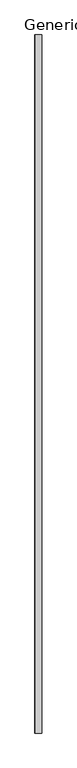
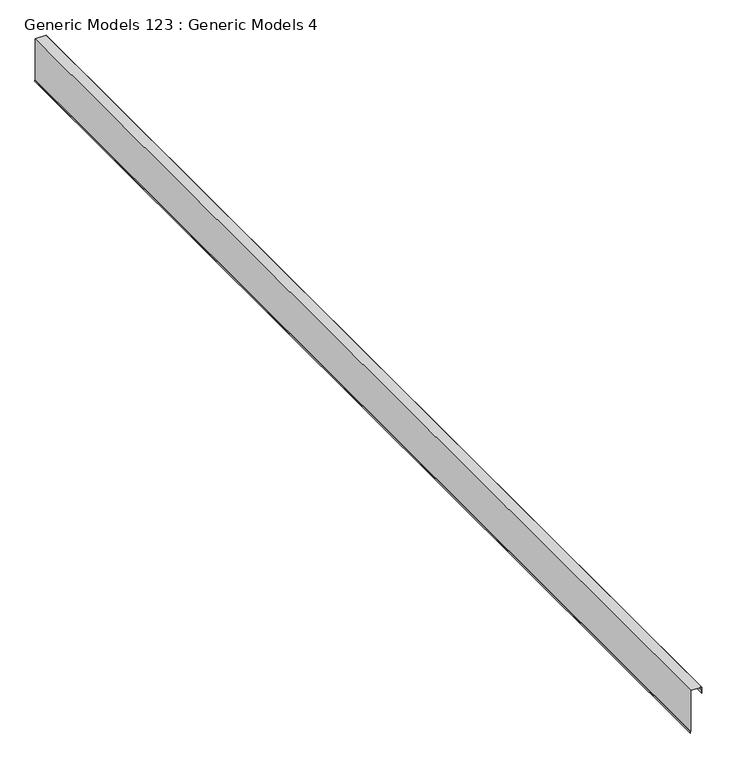
"""IFC4 building model written with IfcOpenShell, lengths in millimetres: proxy geometry, Generic Models 123 : Generic Models 4."""

import ifcopenshell
import ifcopenshell.guid

model = None  # the IFC model being written
_history = None  # IfcOwnerHistory: only IFC2X3 demands one
_inside = {}  # id of a spatial element -> (the spatial element, [elements in it])
_under = {}  # id of a project, library or spatial element -> (it, [spatial elements below it])
_declared = {}  # id of a project -> (the project, [libraries it declares])
_typed = {}  # id of a type object -> (the type object, [elements of that type])
_made_of = {}  # id of a material, layer set ... -> (it, [elements and type objects made of it])


def new_model(schema):
    """Start an empty IFC model of exactly this schema.

    Asked for "IFC4X3", IfcOpenShell would pick the latest addendum, in which some entities
    have other attributes; the version numbers below select the first issue.
    IFC2X3 requires an IfcOwnerHistory on every rooted entity: one is made here for all.
    """
    global model, _history
    if schema == "IFC4X3":
        model = ifcopenshell.file(schema_version=(4, 3, 0, 0))
    else:
        model = ifcopenshell.file(schema=schema)
    _inside.clear()
    _under.clear()
    _declared.clear()
    _typed.clear()
    _made_of.clear()
    _history = None
    if model.schema == "IFC2X3":
        org = make("IfcOrganization", Name="unknown")
        user = make(
            "IfcPersonAndOrganization",
            ThePerson=make("IfcPerson", FamilyName="unknown"),
            TheOrganization=org,
        )
        app = make(
            "IfcApplication",
            ApplicationDeveloper=org,
            Version="unknown",
            ApplicationFullName="unknown",
            ApplicationIdentifier="unknown",
        )
        _history = make(
            "IfcOwnerHistory",
            OwningUser=user,
            OwningApplication=app,
            ChangeAction="ADDED",
            CreationDate=0,
        )
    return model


def make(cls, **values):
    """One entity of the class cls with the attributes given. An attribute that is None is left unset."""
    return model.create_entity(
        cls, **{name: value for name, value in values.items() if value is not None}
    )


def rooted(cls, **values):
    """An entity with a GlobalId (a new one), such as an element, a storey or a relation."""
    return make(cls, GlobalId=ifcopenshell.guid.new(), OwnerHistory=_history, **values)


def si_unit(unit_type, name, prefix=None):
    """IfcSIUnit, for example si_unit("LENGTHUNIT", "METRE", prefix="MILLI")."""
    return make("IfcSIUnit", UnitType=unit_type, Prefix=prefix, Name=name)


def assignment(units):
    """IfcUnitAssignment: the units of a project."""
    return None if units is None else make("IfcUnitAssignment", Units=units)


def point(xyz):
    """IfcCartesianPoint."""
    return None if xyz is None else make("IfcCartesianPoint", Coordinates=xyz)


def direction(xyz):
    """IfcDirection."""
    return None if xyz is None else make("IfcDirection", DirectionRatios=xyz)


def frame(location, z_axis=None, x_axis=None):
    """IfcAxis2Placement3D, a coordinate frame: its origin and axes. An axis left out is left unset."""
    return make(
        "IfcAxis2Placement3D",
        Location=point(location),
        Axis=direction(z_axis),
        RefDirection=direction(x_axis),
    )


def origin():
    """The frame at (0, 0, 0) with its axes left unset."""
    return frame((0.0, 0.0, 0.0))


def place(relative_to, where):
    """IfcLocalPlacement: puts the frame where relative to a parent placement (None: the world)."""
    return make(
        "IfcLocalPlacement", PlacementRelTo=relative_to, RelativePlacement=where
    )


def context(
    kind, dimensions, precision=None, world=None, true_north=None, identifier=None
):
    """IfcGeometricRepresentationContext, for example the 3D "Model" context."""
    return make(
        "IfcGeometricRepresentationContext",
        ContextIdentifier=identifier,
        ContextType=kind,
        CoordinateSpaceDimension=dimensions,
        Precision=precision,
        WorldCoordinateSystem=world,
        TrueNorth=true_north,
    )


def project(units=None, contexts=None):
    """IfcProject with its units and contexts."""
    return rooted(
        "IfcProject",
        Name="project",
        RepresentationContexts=contexts,
        UnitsInContext=assignment(units),
    )


def spatial(cls, under=None, at=None, **own):
    """A site, building, storey or space (cls), placed at a placement, below another one or the project."""
    s = rooted(cls, ObjectPlacement=at, **own)
    if under is not None:
        _under.setdefault(under.id(), (under, []))[1].append(s)
    return s


def polyline(points):
    """IfcPolyline through the points."""
    return make("IfcPolyline", Points=[point(p) for p in points])


def outline(outer, holes=None, kind="AREA"):
    """IfcArbitraryClosedProfileDef: a profile drawn as a closed curve; with holes, ...WithVoids."""
    if holes is None:
        return make("IfcArbitraryClosedProfileDef", ProfileType=kind, OuterCurve=outer)
    return make(
        "IfcArbitraryProfileDefWithVoids",
        ProfileType=kind,
        OuterCurve=outer,
        InnerCurves=holes,
    )


def extrude(swept, where, along, depth):
    """IfcExtrudedAreaSolid: the profile swept, set in the frame where, extruded along a direction by depth."""
    return make(
        "IfcExtrudedAreaSolid",
        SweptArea=swept,
        Position=where,
        ExtrudedDirection=direction(along),
        Depth=depth,
    )


def shape(context_of_items, identifier, shape_type, items):
    """IfcShapeRepresentation: the items that make up one representation, for example the "Body"."""
    return make(
        "IfcShapeRepresentation",
        ContextOfItems=context_of_items,
        RepresentationIdentifier=identifier,
        RepresentationType=shape_type,
        Items=items,
    )


def source(mapping_origin, context_of_items, identifier, shape_type, items):
    """IfcRepresentationMap: a shape defined once, which mapped items show again and again."""
    return make(
        "IfcRepresentationMap",
        MappingOrigin=mapping_origin,
        MappedRepresentation=shape(context_of_items, identifier, shape_type, items),
    )


def transform(
    local_origin,
    x_axis=None,
    y_axis=None,
    z_axis=None,
    scale=None,
    scale2=None,
    scale3=None,
    uniform=True,
):
    """IfcCartesianTransformationOperator3D, or its non-uniform kind. x_axis, y_axis, z_axis: its Axis1, 2, 3."""
    if uniform:
        return make(
            "IfcCartesianTransformationOperator3D",
            Axis1=direction(x_axis),
            Axis2=direction(y_axis),
            LocalOrigin=point(local_origin),
            Scale=scale,
            Axis3=direction(z_axis),
        )
    return make(
        "IfcCartesianTransformationOperator3DnonUniform",
        Axis1=direction(x_axis),
        Axis2=direction(y_axis),
        LocalOrigin=point(local_origin),
        Scale=scale,
        Axis3=direction(z_axis),
        Scale2=scale2,
        Scale3=scale3,
    )


def mapped(mapping_source, mapping_target):
    """IfcMappedItem: shows the shape of a source again, moved by a transform."""
    return make(
        "IfcMappedItem", MappingSource=mapping_source, MappingTarget=mapping_target
    )


def made_of(thing, what):
    """Note that an element or type object is made of a material, layer set ...; save() writes the relation."""
    if what is not None:
        _made_of.setdefault(what.id(), (what, []))[1].append(thing)
    return thing


def element(
    cls,
    number,
    at=None,
    inside=None,
    cuts=None,
    type_object=None,
    material=None,
    context=None,
    identifier="Body",
    shape_type=None,
    held_by="IfcProductDefinitionShape",
    body=None,
    shapes=None,
    **own,
):
    """One element of the class cls, such as IfcWall. Its Tag is "e" and its number.

    at: its placement. inside: the storey or other place that contains it. cuts: it is an
    opening in that element (IfcRelVoidsElement). A single representation is given by context,
    identifier, shape_type and body (its items); several are given by shapes. held_by: the class
    of the entity that holds the representations. save() writes the other relations.
    """
    e = rooted(cls, Tag="e%d" % number, ObjectPlacement=at, **own)
    if body is not None:
        shapes = [shape(context, identifier, shape_type, body)]
    if shapes is not None:
        e.Representation = make(held_by, Representations=shapes)
    if inside is not None:
        _inside.setdefault(inside.id(), (inside, []))[1].append(e)
    if cuts is not None:
        rooted(
            "IfcRelVoidsElement", RelatingBuildingElement=cuts, RelatedOpeningElement=e
        )
    if type_object is not None:
        _typed.setdefault(type_object.id(), (type_object, []))[1].append(e)
    return made_of(e, material)


def aggregate(whole, parts):
    """IfcRelAggregates: a whole, such as a stair, and the parts it consists of."""
    return rooted("IfcRelAggregates", RelatingObject=whole, RelatedObjects=parts)


def save(model, path):
    """Write the relations noted so far, then the file.

    IfcRelAggregates (storeys below a building ...), IfcRelContainedInSpatialStructure (elements
    in a storey), IfcRelDefinesByType, IfcRelAssociatesMaterial and IfcRelDeclares: one each for
    every whole, place, type object, material and project.
    """
    for whole, parts in _under.values():
        aggregate(whole, parts)
    for where, things in _inside.values():
        rooted(
            "IfcRelContainedInSpatialStructure",
            RelatedElements=things,
            RelatingStructure=where,
        )
    for kind, things in _typed.values():
        rooted("IfcRelDefinesByType", RelatedObjects=things, RelatingType=kind)
    for what, things in _made_of.values():
        rooted("IfcRelAssociatesMaterial", RelatedObjects=things, RelatingMaterial=what)
    for by, libraries in _declared.values():
        rooted("IfcRelDeclares", RelatingContext=by, RelatedDefinitions=libraries)
    model.write(path)


def generic_models_123_generic_models_4_3dd0a98e(model_context):
    return source(origin(), model_context, "Body", "SweptSolid", [
        extrude(outline(polyline([(127013.3250789, 7282.3003095), (126974.0744351, 7282.3003095), (126974.0744351, 7283.0940595), (127013.4650384, 7283.0940595), (127020.596979, 7280.4982455), (127078.9254539, 7280.4982455), (127086.571361, 7096.9964748), (126372.7750007, 7096.9964748), (126363.8620646, 7093.7524314), (126344.8395521, 7093.7524314), (126344.8395521, 7094.5461814), (126363.7221051, 7094.5461814), (126372.6350411, 7097.7902248), (127085.7438493, 7097.7902248), (127078.1640881, 7279.7044955), (127020.4570194, 7279.7044955), (127013.3250789, 7282.3003095)])), frame((0.0, -6864.9230338, 0.0), z_axis=(0.0, 1.0, 0.0), x_axis=(0.0, 0.0, 1.0)), (0.0, 0.0, 1.0), 18643.6),
    ])


if __name__ == "__main__":
    model = new_model("IFC4")
    model_context = context("Model", 3, world=origin())
    ifc_project = project(units=[si_unit("LENGTHUNIT", "METRE", prefix="MILLI")], contexts=[model_context])
    site = spatial("IfcSite", under=ifc_project)
    building = spatial("IfcBuilding", under=site)
    placement = place(None, origin())
    generic_models_123_generic_models_4_shape = generic_models_123_generic_models_4_3dd0a98e(model_context)
    element("IfcBuildingElementProxy", 1, Name="Generic Models 123 : Generic Models 4", ObjectType="Generic Models 123 : Generic Models 4", at=placement, inside=building, context=model_context, shape_type="MappedRepresentation", body=[
        mapped(generic_models_123_generic_models_4_shape, transform((0.0, 0.0, 0.0), x_axis=(1.0, 0.0, 0.0), y_axis=(0.0, 1.0, 0.0), z_axis=(0.0, 0.0, 1.0))),
    ])
    save(model, "model.ifc")

# Revit data of these elements
# Element 1 (IfcBuildingElementProxy, "Generic Models 123 : Generic Models 4")
#   Materials on its faces: "_(2) LAYERS NO. 30 ASTM D226 ASPHALT SATURATED ORGANIC FELT"
# Materials
#   "_(2) LAYERS NO. 30 ASTM D226 ASPHALT SATURATED ORGANIC FELT": class "Generic", colour RGB 67 154 161, transparency 0, Cost = 0
